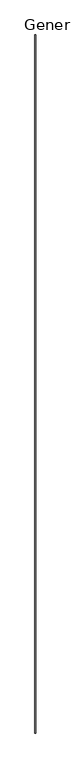
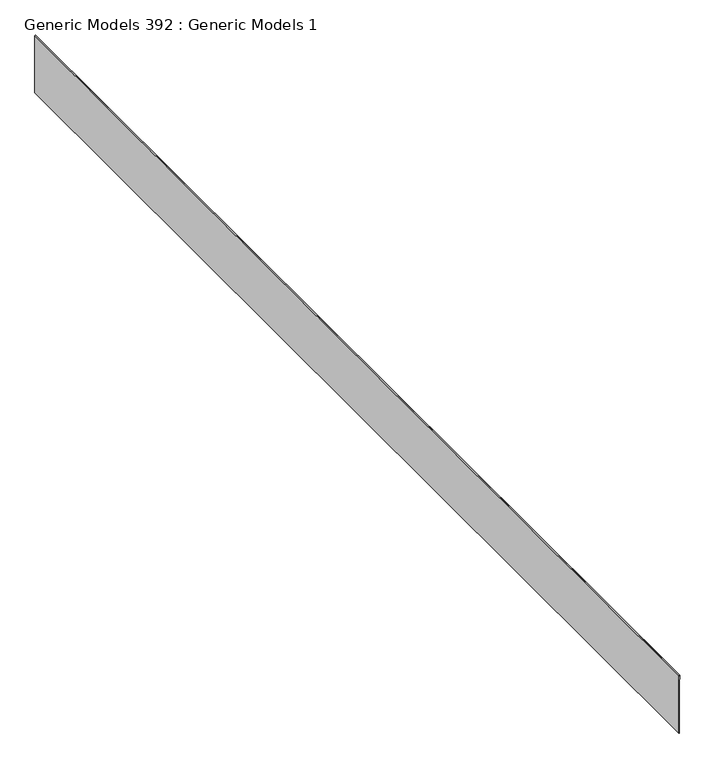
"""IFC4 building model written with IfcOpenShell, lengths in millimetres: proxy geometry, Generic Models 392 : Generic Models 1."""

from ifc_helpers import new_model, si_unit, point, frame, frame_2d, origin, place, context, project, spatial, polyline, circle_curve, trimmed, segment, composite_curve, outline, extrude, source, transform, mapped, element, save


def generic_models_392_generic_models_1_c27d113b(model_context):
    return source(origin(), model_context, "Body", "SweptSolid", [
        extrude(outline(composite_curve([segment(polyline([(129835.519499, -7145.4991734), (129835.519499, -7143.9116734), (130190.6578308, -7143.9116734)]), True, "CONTINUOUS"), segment(trimmed(circle_curve(frame_2d((130190.6578308, -7142.2222912)), 1.6893822), [point((130190.6578308, -7143.9116734))], [point((130190.6578308, -7140.532909))], True, "CARTESIAN"), True, "CONTINUOUS"), segment(polyline([(130190.6578308, -7140.532909), (130168.6587334, -7140.532909), (130168.6587334, -7138.945409), (130190.6578308, -7138.945409)]), True, "CONTINUOUS"), segment(trimmed(circle_curve(frame_2d((130190.6578308, -7142.2222912)), 3.2768822), [point((130190.6578308, -7138.945409))], [point((130190.6578308, -7145.4991734))], False, "CARTESIAN"), True, "CONTINUOUS"), segment(polyline([(130190.6578308, -7145.4991734), (129835.519499, -7145.4991734)]), True, "CONTINUOUS")], self_intersect=False)), frame((0.0, -7039.3472918, 0.0), z_axis=(0.0, 1.0, 0.0), x_axis=(0.0, 0.0, 1.0)), (0.0, 0.0, 1.0), 6575.224258),
    ])


if __name__ == "__main__":
    model = new_model("IFC4")
    model_context = context("Model", 3, world=origin())
    ifc_project = project(units=[si_unit("LENGTHUNIT", "METRE", prefix="MILLI")], contexts=[model_context])
    site = spatial("IfcSite", under=ifc_project)
    building = spatial("IfcBuilding", under=site)
    placement = place(None, origin())
    generic_models_392_generic_models_1_shape = generic_models_392_generic_models_1_c27d113b(model_context)
    element("IfcBuildingElementProxy", 1, Name="Generic Models 392 : Generic Models 1", ObjectType="Generic Models 392 : Generic Models 1", at=placement, inside=building, context=model_context, shape_type="MappedRepresentation", body=[
        mapped(generic_models_392_generic_models_1_shape, transform((0.0, 0.0, 0.0), x_axis=(1.0, 0.0, 0.0), y_axis=(0.0, 1.0, 0.0), z_axis=(0.0, 0.0, 1.0))),
    ])
    save(model, "model.ifc")

# Revit data of these elements
# Element 1 (IfcBuildingElementProxy, "Generic Models 392 : Generic Models 1")
#   Materials on its faces: "_J CLEAT"
# Materials
#   "_J CLEAT": class "Generic", colour RGB 175 175 175, transparency 0, Cost = 0
